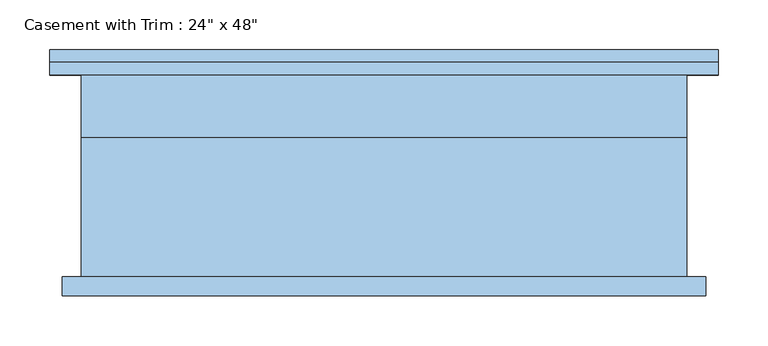
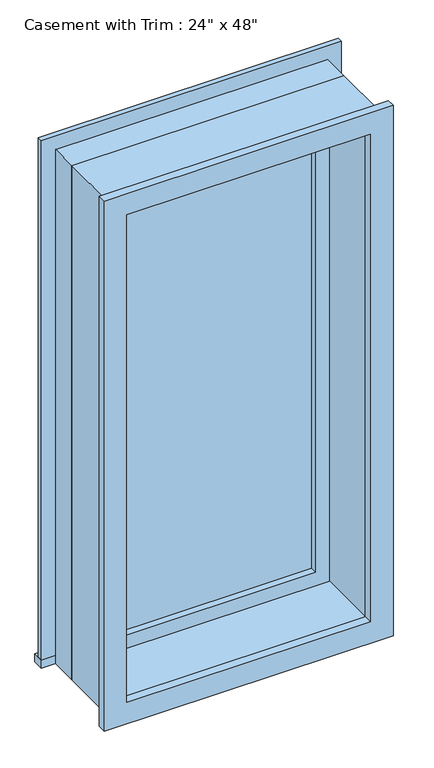
"""IFC4 building model written with IfcOpenShell, lengths in millimetres: window geometry."""

from ifc_helpers import new_model, si_unit, frame, origin, place, context, project, spatial, polyline, outline, extrude, source, transform, mapped, element, save


def window_21430ea7(model_context):
    return source(origin(), model_context, "Body", "SweptSolid", [
        extrude(outline(polyline([(-336.55, 127.0), (336.55, 127.0), (336.55, 101.6), (-336.55, 101.6), (-336.55, 127.0)])), frame((0.0, 0.0, 914.4), z_axis=(0.0, 0.0, 1.0), x_axis=(1.0, 0.0, 0.0)), (0.0, 0.0, 1.0), 19.05),
        extrude(outline(polyline([(2114.55, -285.75), (2114.55, 285.75), (933.45, 285.75), (933.45, 336.55), (2165.35, 336.55), (2165.35, -336.55), (933.45, -336.55), (933.45, -285.75), (2114.55, -285.75)])), frame((0.0, 101.6, 0.0), z_axis=(0.0, 1.0, 0.0), x_axis=(0.0, 0.0, 1.0)), (0.0, 0.0, 1.0), 12.7),
        extrude(outline(polyline([(2152.65, 323.85), (2152.65, -323.85), (895.35, -323.85), (895.35, 323.85), (2152.65, 323.85)]), holes=[polyline([(2101.85, 273.05), (946.15, 273.05), (946.15, -273.05), (2101.85, -273.05), (2101.85, 273.05)])]), frame((0.0, -120.65, 0.0), z_axis=(0.0, 1.0, 0.0), x_axis=(0.0, 0.0, 1.0)), (0.0, 0.0, 1.0), 19.05),
        extrude(outline(polyline([(241.3, 53.975), (-241.3, 53.975), (-241.3, 66.675), (241.3, 66.675), (241.3, 53.975)])), frame((0.0, 0.0, 977.9), z_axis=(0.0, 0.0, 1.0), x_axis=(1.0, 0.0, 0.0)), (0.0, 0.0, 1.0), 1092.2),
        extrude(outline(polyline([(2114.55, -285.75), (933.45, -285.75), (933.45, 285.75), (2114.55, 285.75), (2114.55, -285.75)]), holes=[polyline([(2070.1, -241.3), (2070.1, 241.3), (977.9, 241.3), (977.9, -241.3), (2070.1, -241.3)])]), frame((0.0, 38.1, 0.0), z_axis=(0.0, 1.0, 0.0), x_axis=(0.0, 0.0, 1.0)), (0.0, 0.0, 1.0), 44.45),
        extrude(outline(polyline([(2133.6, -304.8), (914.4, -304.8), (914.4, 304.8), (2133.6, 304.8), (2133.6, -304.8)]), holes=[polyline([(2101.85, -273.05), (2101.85, 273.05), (946.15, 273.05), (946.15, -273.05), (2101.85, -273.05)])]), frame((0.0, -101.6, 0.0), z_axis=(0.0, 1.0, 0.0), x_axis=(0.0, 0.0, 1.0)), (0.0, 0.0, 1.0), 139.7),
        extrude(outline(polyline([(2133.6, 304.8), (2133.6, -304.8), (914.4, -304.8), (914.4, 304.8), (2133.6, 304.8)]), holes=[polyline([(2114.55, 285.75), (933.45, 285.75), (933.45, -285.75), (2114.55, -285.75), (2114.55, 285.75)])]), frame((0.0, 38.1, 0.0), z_axis=(0.0, 1.0, 0.0), x_axis=(0.0, 0.0, 1.0)), (0.0, 0.0, 1.0), 63.5),
    ])


if __name__ == "__main__":
    model = new_model("IFC4")
    model_context = context("Model", 3, world=origin())
    ifc_project = project(units=[si_unit("LENGTHUNIT", "METRE", prefix="MILLI")], contexts=[model_context])
    site = spatial("IfcSite", under=ifc_project)
    building = spatial("IfcBuilding", under=site)
    placement = place(None, origin())
    window_shape = window_21430ea7(model_context)
    element("IfcWindow", 1, ObjectType="Casement with Trim : 24\" x 48\"", at=placement, inside=building, context=model_context, shape_type="MappedRepresentation", body=[
        mapped(window_shape, transform((0.0, 0.0, 0.0), x_axis=(1.0, 0.0, 0.0), y_axis=(0.0, 1.0, 0.0), z_axis=(0.0, 0.0, 1.0))),
    ])
    save(model, "model.ifc")

# Revit data of these elements
# Type "Casement with Trim : 24\" x 48\""
#   Type Mark = "39"
#   Assembly Code = "B2020100"
#   Height = 4' - 0"
#   Default Sill Height = 3' - 0"
#   Trim Projection - Ext. = 0' - 0 1/2"
#   Trim Projection - Int. = 0' - 0 3/4"
#   Trim Width - Exterior = 0' - 2"
#   Trim Width - Interior = 0' - 2"
#   Width = 2' - 0"
#   Window Inset = 0' - 0 3/4"
#   Glass Pane Material = Glass
#   Sash Material = Sash
#   Trim Exterior Material = Trim
#   Trim Interior Material = Trim
#   Wall Closure = (empty or 0)
# Element 1 (IfcWindow, "Casement with Trim : 24\" x 48\"")
#   Materials on its faces: "Sash", "Trim", "Glass"
# Materials
#   "Glass": class "Glass", colour RGB 0 128 192, transparency 0.75
#   "Sash": class "Wood", colour RGB 224 178 126, transparency 0
#   "Trim": class "Wood", colour RGB 224 178 126, transparency 0
